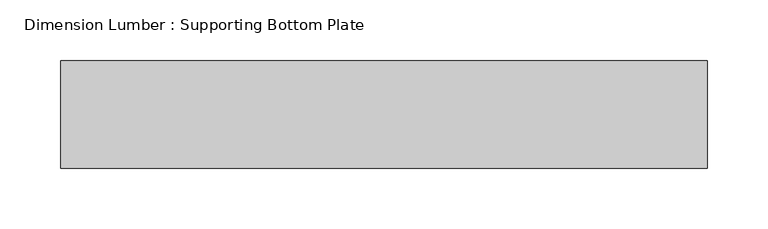
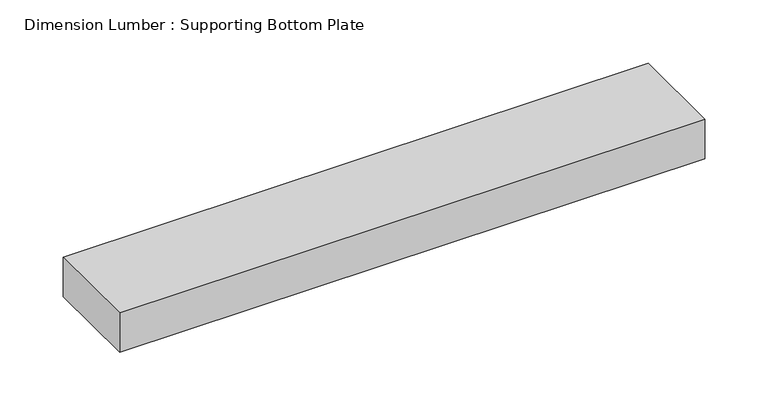
"""IFC4 building model written with IfcOpenShell, lengths in millimetres: beam geometry, Dimension Lumber : Supporting Bottom Plate."""

from ifc_helpers import new_model, si_unit, frame, origin, place, context, project, spatial, polyline, outline, extrude, source, transform, mapped, element, save


def dimension_lumber_supporting_bottom_plate_a6d88285(model_context):
    return source(origin(), model_context, "Body", "SweptSolid", [
        extrude(outline(polyline([(682.325, 44.45), (1216.325, 44.45), (1216.325, -44.45), (682.325, -44.45), (682.325, 44.45)])), frame((0.0, 0.0, -19.05), z_axis=(0.0, 0.0, 1.0), x_axis=(1.0, 0.0, 0.0)), (0.0, 0.0, 1.0), 38.1),
    ])


if __name__ == "__main__":
    model = new_model("IFC4")
    model_context = context("Model", 3, world=origin())
    ifc_project = project(units=[si_unit("LENGTHUNIT", "METRE", prefix="MILLI")], contexts=[model_context])
    site = spatial("IfcSite", under=ifc_project)
    building = spatial("IfcBuilding", under=site)
    placement = place(None, origin())
    dimension_lumber_supporting_bottom_plate_shape = dimension_lumber_supporting_bottom_plate_a6d88285(model_context)
    element("IfcBeam", 1, ObjectType="Dimension Lumber : Supporting Bottom Plate", at=placement, inside=building, context=model_context, shape_type="MappedRepresentation", body=[
        mapped(dimension_lumber_supporting_bottom_plate_shape, transform((0.0, 0.0, 0.0), x_axis=(1.0, 0.0, 0.0), y_axis=(0.0, 1.0, 0.0), z_axis=(0.0, 0.0, 1.0))),
    ])
    save(model, "model.ifc")

# Revit data of these elements
# Type "Dimension Lumber : Supporting Bottom Plate"
#   Assembly Code = "B10"
#   A = 0.0364583 SF
#   Length [instance default] = 5' - 0"
#   b = 0' - 3 1/2"
#   d = 0' - 1 1/2"
#   Structural Material [instance default] = Softwood, Lumber
# Element 1 (IfcBeam, "Dimension Lumber : Supporting Bottom Plate")
#   Structural Material = Douglas Fir #2
#   Materials on its faces: "Douglas Fir #2"
# Materials
#   "Softwood, Lumber": class "Wood", colour RGB 223 192 134, transparency 0, Description = "Pinus Echinata", Cost = 0
#   "Douglas Fir #2": class "Wood", colour RGB 223 192 134, transparency 0, Description = "Pinus Echinata", Cost = 0
